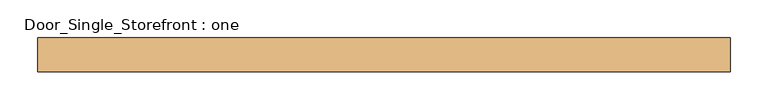
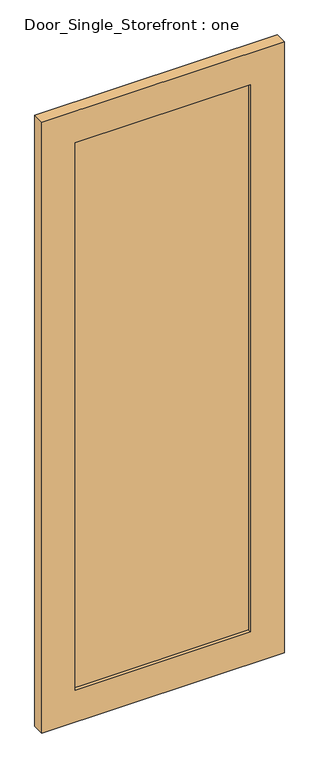
"""IFC4 building model written with IfcOpenShell, lengths in millimetres: door geometry, Door_Single_Storefront : one."""

from ifc_helpers import new_model, si_unit, frame, origin, place, context, project, spatial, polyline, outline, extrude, source, transform, mapped, element, save


def door_single_storefront_one_2492f337(model_context):
    return source(origin(), model_context, "Body", "SweptSolid", [
        extrude(outline(polyline([(330.2, -6.35), (-330.2, -6.35), (-330.2, 12.7), (330.2, 12.7), (330.2, -6.35)])), frame((0.0, 0.0, 127.0), z_axis=(0.0, 0.0, 1.0), x_axis=(1.0, 0.0, 0.0)), (0.0, 0.0, 1.0), 2178.05),
        extrude(outline(polyline([(2432.05, -457.2), (0.0, -457.2), (0.0, 457.2), (2432.05, 457.2), (2432.05, -457.2)]), holes=[polyline([(127.0, 330.2), (127.0, -330.2), (2305.05, -330.2), (2305.05, 330.2), (127.0, 330.2)])]), frame((0.0, -19.05, 0.0), z_axis=(0.0, 1.0, 0.0), x_axis=(0.0, 0.0, 1.0)), (0.0, 0.0, 1.0), 44.45),
    ])


if __name__ == "__main__":
    model = new_model("IFC4")
    model_context = context("Model", 3, world=origin())
    ifc_project = project(units=[si_unit("LENGTHUNIT", "METRE", prefix="MILLI")], contexts=[model_context])
    site = spatial("IfcSite", under=ifc_project)
    building = spatial("IfcBuilding", under=site)
    placement = place(None, origin())
    door_single_storefront_one_shape = door_single_storefront_one_2492f337(model_context)
    element("IfcDoor", 1, ObjectType="Door_Single_Storefront : one", at=placement, inside=building, context=model_context, shape_type="MappedRepresentation", body=[
        mapped(door_single_storefront_one_shape, transform((0.0, 0.0, 0.0), x_axis=(1.0, 0.0, 0.0), y_axis=(0.0, 1.0, 0.0), z_axis=(0.0, 0.0, 1.0))),
    ])
    save(model, "model.ifc")

# Revit data of these elements
# Type "Door_Single_Storefront : one"
#   Type Mark = "27"
#   Analytic Construction = "<None>"
#   Stile_Width = 0' - 5"
#   Door_Thickness = 0' - 1 3/4"
#   Door_Offset = 0' - 1"
#   Glass_Material = SAFETY GLAZING
#   Frame_Material = INTERIOR GRADE ALUMINUM STOREFRONT W/ SAFETY GLAZING
#   Function = (empty or 0)
# Element 1 (IfcDoor, "Door_Single_Storefront : one")
#   Materials on its faces: "INTERIOR GRADE ALUMINUM STOREFRONT W/ SAFETY GLAZING", "SAFETY GLAZING"
# Materials
#   "SAFETY GLAZING": class "Glass", colour RGB 142 168 196, transparency 0.75, Description = "Soda Lime Glass", Cost = 0
#   "INTERIOR GRADE ALUMINUM STOREFRONT W/ SAFETY GLAZING": class "Metal", colour RGB 226 226 226, transparency 0, Description = "Aluminum 6061", Cost = 0
